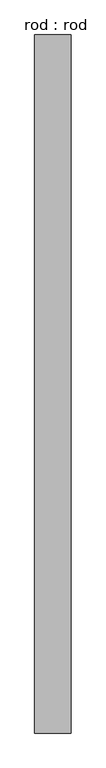
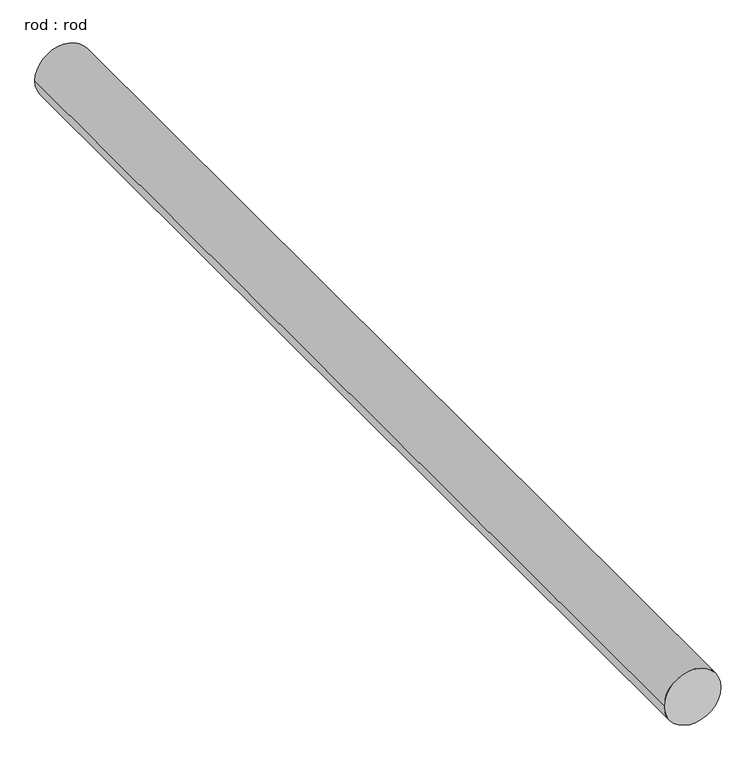
"""IFC4 building model written with IfcOpenShell, lengths in millimetres: proxy geometry, rod : rod."""

import ifcopenshell
import ifcopenshell.guid

model = None  # the IFC model being written
_history = None  # IfcOwnerHistory: only IFC2X3 demands one
_inside = {}  # id of a spatial element -> (the spatial element, [elements in it])
_under = {}  # id of a project, library or spatial element -> (it, [spatial elements below it])
_declared = {}  # id of a project -> (the project, [libraries it declares])
_typed = {}  # id of a type object -> (the type object, [elements of that type])
_made_of = {}  # id of a material, layer set ... -> (it, [elements and type objects made of it])


def new_model(schema):
    """Start an empty IFC model of exactly this schema.

    Asked for "IFC4X3", IfcOpenShell would pick the latest addendum, in which some entities
    have other attributes; the version numbers below select the first issue.
    IFC2X3 requires an IfcOwnerHistory on every rooted entity: one is made here for all.
    """
    global model, _history
    if schema == "IFC4X3":
        model = ifcopenshell.file(schema_version=(4, 3, 0, 0))
    else:
        model = ifcopenshell.file(schema=schema)
    _inside.clear()
    _under.clear()
    _declared.clear()
    _typed.clear()
    _made_of.clear()
    _history = None
    if model.schema == "IFC2X3":
        org = make("IfcOrganization", Name="unknown")
        user = make(
            "IfcPersonAndOrganization",
            ThePerson=make("IfcPerson", FamilyName="unknown"),
            TheOrganization=org,
        )
        app = make(
            "IfcApplication",
            ApplicationDeveloper=org,
            Version="unknown",
            ApplicationFullName="unknown",
            ApplicationIdentifier="unknown",
        )
        _history = make(
            "IfcOwnerHistory",
            OwningUser=user,
            OwningApplication=app,
            ChangeAction="ADDED",
            CreationDate=0,
        )
    return model


def make(cls, **values):
    """One entity of the class cls with the attributes given. An attribute that is None is left unset."""
    return model.create_entity(
        cls, **{name: value for name, value in values.items() if value is not None}
    )


def rooted(cls, **values):
    """An entity with a GlobalId (a new one), such as an element, a storey or a relation."""
    return make(cls, GlobalId=ifcopenshell.guid.new(), OwnerHistory=_history, **values)


def si_unit(unit_type, name, prefix=None):
    """IfcSIUnit, for example si_unit("LENGTHUNIT", "METRE", prefix="MILLI")."""
    return make("IfcSIUnit", UnitType=unit_type, Prefix=prefix, Name=name)


def assignment(units):
    """IfcUnitAssignment: the units of a project."""
    return None if units is None else make("IfcUnitAssignment", Units=units)


def point(xyz):
    """IfcCartesianPoint."""
    return None if xyz is None else make("IfcCartesianPoint", Coordinates=xyz)


def direction(xyz):
    """IfcDirection."""
    return None if xyz is None else make("IfcDirection", DirectionRatios=xyz)


def frame(location, z_axis=None, x_axis=None):
    """IfcAxis2Placement3D, a coordinate frame: its origin and axes. An axis left out is left unset."""
    return make(
        "IfcAxis2Placement3D",
        Location=point(location),
        Axis=direction(z_axis),
        RefDirection=direction(x_axis),
    )


def frame_2d(location, x_axis=None):
    """IfcAxis2Placement2D, a coordinate frame in the plane: its origin and x axis."""
    return make(
        "IfcAxis2Placement2D", Location=point(location), RefDirection=direction(x_axis)
    )


def origin():
    """The frame at (0, 0, 0) with its axes left unset."""
    return frame((0.0, 0.0, 0.0))


def place(relative_to, where):
    """IfcLocalPlacement: puts the frame where relative to a parent placement (None: the world)."""
    return make(
        "IfcLocalPlacement", PlacementRelTo=relative_to, RelativePlacement=where
    )


def context(
    kind, dimensions, precision=None, world=None, true_north=None, identifier=None
):
    """IfcGeometricRepresentationContext, for example the 3D "Model" context."""
    return make(
        "IfcGeometricRepresentationContext",
        ContextIdentifier=identifier,
        ContextType=kind,
        CoordinateSpaceDimension=dimensions,
        Precision=precision,
        WorldCoordinateSystem=world,
        TrueNorth=true_north,
    )


def project(units=None, contexts=None):
    """IfcProject with its units and contexts."""
    return rooted(
        "IfcProject",
        Name="project",
        RepresentationContexts=contexts,
        UnitsInContext=assignment(units),
    )


def spatial(cls, under=None, at=None, **own):
    """A site, building, storey or space (cls), placed at a placement, below another one or the project."""
    s = rooted(cls, ObjectPlacement=at, **own)
    if under is not None:
        _under.setdefault(under.id(), (under, []))[1].append(s)
    return s


def circle_curve(where, radius):
    """IfcCircle in the frame where."""
    return make("IfcCircle", Position=where, Radius=radius)


def trimmed(basis, trim1, trim2, sense, master):
    """IfcTrimmedCurve: the piece of a basis curve between two trims."""
    return make(
        "IfcTrimmedCurve",
        BasisCurve=basis,
        Trim1=trim1,
        Trim2=trim2,
        SenseAgreement=sense,
        MasterRepresentation=master,
    )


def segment(curve, same_sense, transition):
    """IfcCompositeCurveSegment."""
    return make(
        "IfcCompositeCurveSegment",
        Transition=transition,
        SameSense=same_sense,
        ParentCurve=curve,
    )


def composite_curve(segments, self_intersect=None):
    """IfcCompositeCurve: segments joined end to end."""
    return make("IfcCompositeCurve", Segments=segments, SelfIntersect=self_intersect)


def outline(outer, holes=None, kind="AREA"):
    """IfcArbitraryClosedProfileDef: a profile drawn as a closed curve; with holes, ...WithVoids."""
    if holes is None:
        return make("IfcArbitraryClosedProfileDef", ProfileType=kind, OuterCurve=outer)
    return make(
        "IfcArbitraryProfileDefWithVoids",
        ProfileType=kind,
        OuterCurve=outer,
        InnerCurves=holes,
    )


def extrude(swept, where, along, depth):
    """IfcExtrudedAreaSolid: the profile swept, set in the frame where, extruded along a direction by depth."""
    return make(
        "IfcExtrudedAreaSolid",
        SweptArea=swept,
        Position=where,
        ExtrudedDirection=direction(along),
        Depth=depth,
    )


def shape(context_of_items, identifier, shape_type, items):
    """IfcShapeRepresentation: the items that make up one representation, for example the "Body"."""
    return make(
        "IfcShapeRepresentation",
        ContextOfItems=context_of_items,
        RepresentationIdentifier=identifier,
        RepresentationType=shape_type,
        Items=items,
    )


def source(mapping_origin, context_of_items, identifier, shape_type, items):
    """IfcRepresentationMap: a shape defined once, which mapped items show again and again."""
    return make(
        "IfcRepresentationMap",
        MappingOrigin=mapping_origin,
        MappedRepresentation=shape(context_of_items, identifier, shape_type, items),
    )


def transform(
    local_origin,
    x_axis=None,
    y_axis=None,
    z_axis=None,
    scale=None,
    scale2=None,
    scale3=None,
    uniform=True,
):
    """IfcCartesianTransformationOperator3D, or its non-uniform kind. x_axis, y_axis, z_axis: its Axis1, 2, 3."""
    if uniform:
        return make(
            "IfcCartesianTransformationOperator3D",
            Axis1=direction(x_axis),
            Axis2=direction(y_axis),
            LocalOrigin=point(local_origin),
            Scale=scale,
            Axis3=direction(z_axis),
        )
    return make(
        "IfcCartesianTransformationOperator3DnonUniform",
        Axis1=direction(x_axis),
        Axis2=direction(y_axis),
        LocalOrigin=point(local_origin),
        Scale=scale,
        Axis3=direction(z_axis),
        Scale2=scale2,
        Scale3=scale3,
    )


def mapped(mapping_source, mapping_target):
    """IfcMappedItem: shows the shape of a source again, moved by a transform."""
    return make(
        "IfcMappedItem", MappingSource=mapping_source, MappingTarget=mapping_target
    )


def made_of(thing, what):
    """Note that an element or type object is made of a material, layer set ...; save() writes the relation."""
    if what is not None:
        _made_of.setdefault(what.id(), (what, []))[1].append(thing)
    return thing


def element(
    cls,
    number,
    at=None,
    inside=None,
    cuts=None,
    type_object=None,
    material=None,
    context=None,
    identifier="Body",
    shape_type=None,
    held_by="IfcProductDefinitionShape",
    body=None,
    shapes=None,
    **own,
):
    """One element of the class cls, such as IfcWall. Its Tag is "e" and its number.

    at: its placement. inside: the storey or other place that contains it. cuts: it is an
    opening in that element (IfcRelVoidsElement). A single representation is given by context,
    identifier, shape_type and body (its items); several are given by shapes. held_by: the class
    of the entity that holds the representations. save() writes the other relations.
    """
    e = rooted(cls, Tag="e%d" % number, ObjectPlacement=at, **own)
    if body is not None:
        shapes = [shape(context, identifier, shape_type, body)]
    if shapes is not None:
        e.Representation = make(held_by, Representations=shapes)
    if inside is not None:
        _inside.setdefault(inside.id(), (inside, []))[1].append(e)
    if cuts is not None:
        rooted(
            "IfcRelVoidsElement", RelatingBuildingElement=cuts, RelatedOpeningElement=e
        )
    if type_object is not None:
        _typed.setdefault(type_object.id(), (type_object, []))[1].append(e)
    return made_of(e, material)


def aggregate(whole, parts):
    """IfcRelAggregates: a whole, such as a stair, and the parts it consists of."""
    return rooted("IfcRelAggregates", RelatingObject=whole, RelatedObjects=parts)


def save(model, path):
    """Write the relations noted so far, then the file.

    IfcRelAggregates (storeys below a building ...), IfcRelContainedInSpatialStructure (elements
    in a storey), IfcRelDefinesByType, IfcRelAssociatesMaterial and IfcRelDeclares: one each for
    every whole, place, type object, material and project.
    """
    for whole, parts in _under.values():
        aggregate(whole, parts)
    for where, things in _inside.values():
        rooted(
            "IfcRelContainedInSpatialStructure",
            RelatedElements=things,
            RelatingStructure=where,
        )
    for kind, things in _typed.values():
        rooted("IfcRelDefinesByType", RelatedObjects=things, RelatingType=kind)
    for what, things in _made_of.values():
        rooted("IfcRelAssociatesMaterial", RelatedObjects=things, RelatingMaterial=what)
    for by, libraries in _declared.values():
        rooted("IfcRelDeclares", RelatingContext=by, RelatedDefinitions=libraries)
    model.write(path)


def rod_rod_0ac2e2dc(model_context):
    return source(origin(), model_context, "Body", "SweptSolid", [
        extrude(outline(composite_curve([segment(trimmed(circle_curve(frame_2d((0.0108462, 0.0)), 200.0), [point((0.0108462, 200.0))], [point((0.0108462, -200.0))], False, "CARTESIAN"), True, "CONTINUOUS"), segment(trimmed(circle_curve(frame_2d((0.0108462, 0.0)), 200.0), [point((0.0108462, -200.0))], [point((0.0108462, 200.0))], False, "CARTESIAN"), True, "CONTINUOUS")], self_intersect=False)), frame((0.0, 260.8438246, 0.0), z_axis=(0.0, 1.0, 0.0), x_axis=(0.0, 0.0, 1.0)), (0.0, 0.0, 1.0), 7663.7695814),
    ])


if __name__ == "__main__":
    model = new_model("IFC4")
    model_context = context("Model", 3, world=origin())
    ifc_project = project(units=[si_unit("LENGTHUNIT", "METRE", prefix="MILLI")], contexts=[model_context])
    site = spatial("IfcSite", under=ifc_project)
    building = spatial("IfcBuilding", under=site)
    placement = place(None, origin())
    rod_rod_shape = rod_rod_0ac2e2dc(model_context)
    element("IfcBuildingElementProxy", 1, Name="rod : rod", ObjectType="rod : rod", at=placement, inside=building, context=model_context, shape_type="MappedRepresentation", body=[
        mapped(rod_rod_shape, transform((0.0, 0.0, 0.0), x_axis=(1.0, 0.0, 0.0), y_axis=(0.0, 1.0, 0.0), z_axis=(0.0, 0.0, 1.0))),
    ])
    save(model, "model.ifc")

# Revit data of these elements
# Type "rod : rod"
#   Default Elevation = 0
